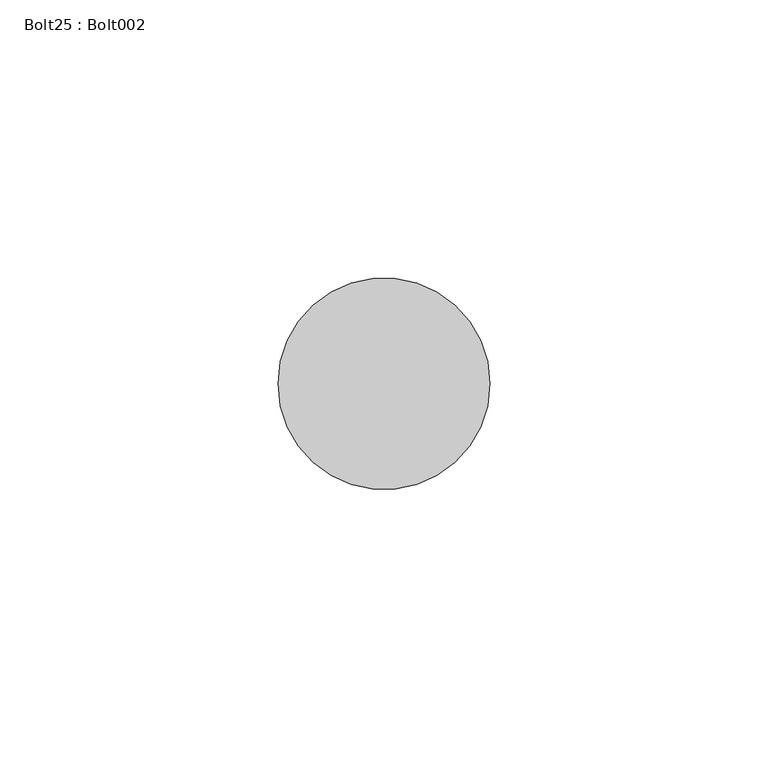
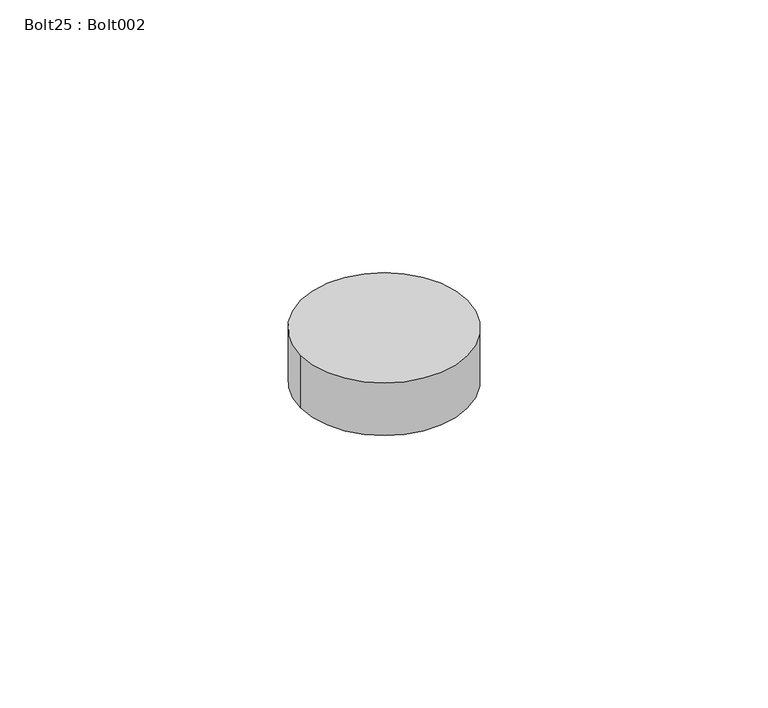
"""IFC4 building model written with IfcOpenShell, lengths in millimetres: proxy geometry, Bolt25 : Bolt002."""

from ifc_helpers import new_model, si_unit, point, frame, frame_2d, origin, place, context, project, spatial, circle_curve, trimmed, segment, composite_curve, outline, extrude, source, transform, mapped, element, save


def bolt25_bolt002_17bbbc31(model_context):
    return source(origin(), model_context, "Body", "SweptSolid", [
        extrude(outline(composite_curve([segment(trimmed(circle_curve(frame_2d((5172.3828124, 1896.5882072)), 19.05), [point((5153.3328124, 1896.5882072))], [point((5191.4328124, 1896.5882072))], False, "CARTESIAN"), True, "CONTINUOUS"), segment(trimmed(circle_curve(frame_2d((5172.3828124, 1896.5882072)), 19.05), [point((5191.4328124, 1896.5882072))], [point((5153.3328124, 1896.5882072))], False, "CARTESIAN"), True, "CONTINUOUS")], self_intersect=False)), frame((0.0, 0.0, 36709.0959962), z_axis=(0.0, 0.0, 1.0), x_axis=(1.0, 0.0, 0.0)), (0.0, 0.0, 1.0), 12.7),
    ])


if __name__ == "__main__":
    model = new_model("IFC4")
    model_context = context("Model", 3, world=origin())
    ifc_project = project(units=[si_unit("LENGTHUNIT", "METRE", prefix="MILLI")], contexts=[model_context])
    site = spatial("IfcSite", under=ifc_project)
    building = spatial("IfcBuilding", under=site)
    placement = place(None, origin())
    bolt25_bolt002_shape = bolt25_bolt002_17bbbc31(model_context)
    element("IfcBuildingElementProxy", 1, Name="Bolt25 : Bolt002", ObjectType="Bolt25 : Bolt002", at=placement, inside=building, context=model_context, shape_type="MappedRepresentation", body=[
        mapped(bolt25_bolt002_shape, transform((0.0, 0.0, 0.0), x_axis=(1.0, 0.0, 0.0), y_axis=(0.0, 1.0, 0.0), z_axis=(0.0, 0.0, 1.0))),
    ])
    save(model, "model.ifc")

# Revit data of these elements
# Type "Bolt25 : Bolt002"
#   NameOverride = "Bolt002"
# Element 1 (IfcBuildingElementProxy, "Bolt25 : Bolt002")
#   Materials on its faces: "STEEL ANGLE AND ANCHOR BOLT (SEE STRUCT. DWGS)"
# Materials
#   "STEEL ANGLE AND ANCHOR BOLT (SEE STRUCT. DWGS)": class "Unassigned", colour RGB 128 128 128, transparency 0, Cost = 0
